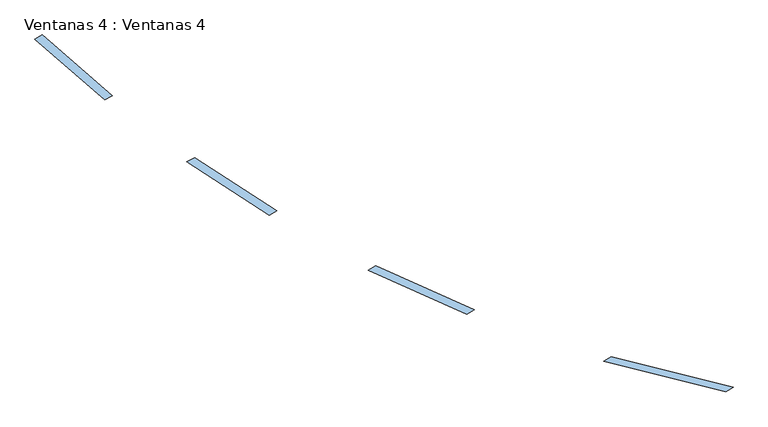
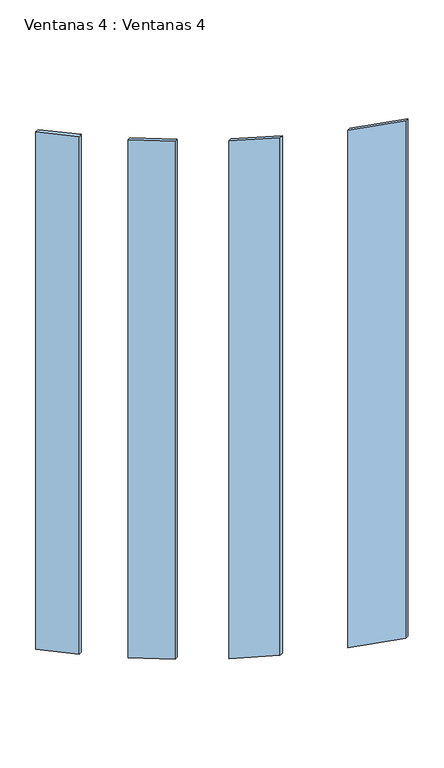
"""IFC4 building model written with IfcOpenShell, lengths in millimetres: window geometry, Ventanas 4 : Ventanas 4."""

from ifc_helpers import new_model, si_unit, frame, origin, place, context, project, spatial, polyline, outline, extrude, source, transform, mapped, element, save


def ventanas_4_ventanas_4_bcc6f8dd(model_context):
    return source(origin(), model_context, "Body", "SweptSolid", [
        extrude(outline(polyline([(-7534.4171481, 5113.3905673), (-7551.7376561, 5103.3905673), (-7711.3769482, 5242.1628867), (-7694.0564401, 5252.1628867), (-7534.4171481, 5113.3905673)])), frame((0.0, 0.0, 6206.6549752), z_axis=(0.0, 0.0, 1.0), x_axis=(1.0, 0.0, 0.0)), (0.0, 0.0, 1.0), 3027.3080819),
        extrude(outline(polyline([(-7157.5445793, 4849.0025368), (-7174.8650874, 4839.0025368), (-7363.117484, 4961.2550726), (-7345.7969759, 4971.2550726), (-7157.5445793, 4849.0025368)])), frame((0.0, 0.0, 6206.6549752), z_axis=(0.0, 0.0, 1.0), x_axis=(1.0, 0.0, 0.0)), (0.0, 0.0, 1.0), 3027.3080819),
        extrude(outline(polyline([(-6704.9684728, 4622.770308), (-6722.2889809, 4612.770308), (-6948.1298381, 4713.3211359), (-6930.8093301, 4723.3211359), (-6704.9684728, 4622.770308)])), frame((0.0, 0.0, 6206.6549752), z_axis=(0.0, 0.0, 1.0), x_axis=(1.0, 0.0, 0.0)), (0.0, 0.0, 1.0), 3027.3080819),
        extrude(outline(polyline([(-6112.3476086, 4445.253587), (-6129.6681167, 4435.253587), (-6409.0272283, 4504.9056363), (-6391.7067202, 4514.9056363), (-6112.3476086, 4445.253587)])), frame((0.0, 0.0, 6206.6549752), z_axis=(0.0, 0.0, 1.0), x_axis=(1.0, 0.0, 0.0)), (0.0, 0.0, 1.0), 3027.3080819),
    ])


if __name__ == "__main__":
    model = new_model("IFC4")
    model_context = context("Model", 3, world=origin())
    ifc_project = project(units=[si_unit("LENGTHUNIT", "METRE", prefix="MILLI")], contexts=[model_context])
    site = spatial("IfcSite", under=ifc_project)
    building = spatial("IfcBuilding", under=site)
    placement = place(None, origin())
    ventanas_4_ventanas_4_shape = ventanas_4_ventanas_4_bcc6f8dd(model_context)
    element("IfcWindow", 1, ObjectType="Ventanas 4 : Ventanas 4", at=placement, inside=building, context=model_context, shape_type="MappedRepresentation", body=[
        mapped(ventanas_4_ventanas_4_shape, transform((0.0, 0.0, 0.0), x_axis=(1.0, 0.0, 0.0), y_axis=(0.0, 1.0, 0.0), z_axis=(0.0, 0.0, 1.0))),
    ])
    save(model, "model.ifc")

# Revit data of these elements
# Type "Ventanas 4 : Ventanas 4"
#   Type Mark = "30"
# Element 1 (IfcWindow, "Ventanas 4 : Ventanas 4")
#   Materials on its faces: "VIDRIO"
# Materials
#   "VIDRIO": class "Genérico", colour RGB 120 120 120, transparency 0, Cost = 0
